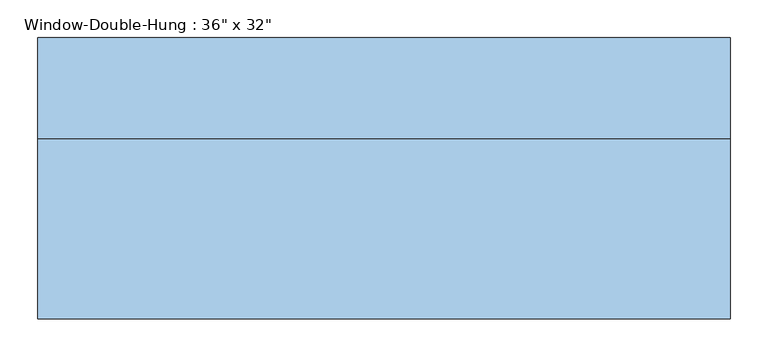
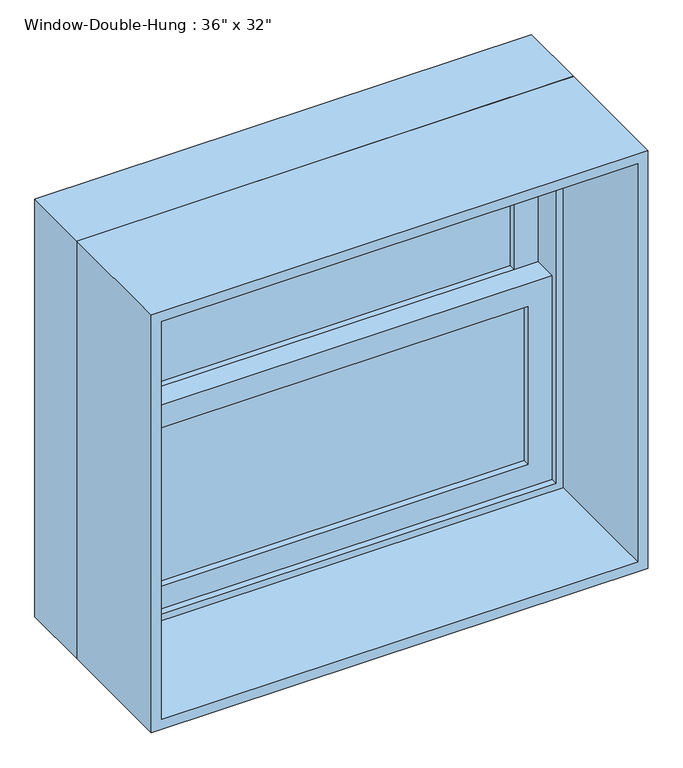
"""IFC4 building model written with IfcOpenShell, lengths in millimetres: window geometry."""

from ifc_helpers import new_model, si_unit, frame, origin, place, context, project, spatial, polyline, outline, extrude, source, transform, mapped, element, save


def window_e999161c(model_context):
    return source(origin(), model_context, "Body", "SweptSolid", [
        extrude(outline(polyline([(381.0, 106.3625), (381.0, 100.0125), (-381.0, 100.0125), (-381.0, 106.3625), (381.0, 106.3625)])), frame((0.0, 0.0, 990.6), z_axis=(0.0, 0.0, 1.0), x_axis=(1.0, 0.0, 0.0)), (0.0, 0.0, 1.0), 307.975),
        extrude(outline(polyline([(-381.0, 93.6625), (381.0, 93.6625), (381.0, 87.3125), (-381.0, 87.3125), (-381.0, 93.6625)])), frame((0.0, 0.0, 990.6), z_axis=(0.0, 0.0, 1.0), x_axis=(1.0, 0.0, 0.0)), (0.0, 0.0, 1.0), 307.975),
        extrude(outline(polyline([(381.0, 150.8125), (381.0, 144.4625), (-381.0, 144.4625), (-381.0, 150.8125), (381.0, 150.8125)])), frame((0.0, 0.0, 1343.025), z_axis=(0.0, 0.0, 1.0), x_axis=(1.0, 0.0, 0.0)), (0.0, 0.0, 1.0), 307.975),
        extrude(outline(polyline([(-381.0, 138.1125), (381.0, 138.1125), (381.0, 131.7625), (-381.0, 131.7625), (-381.0, 138.1125)])), frame((0.0, 0.0, 1343.025), z_axis=(0.0, 0.0, 1.0), x_axis=(1.0, 0.0, 0.0)), (0.0, 0.0, 1.0), 307.975),
        extrude(outline(polyline([(1343.025, -425.45), (946.15, -425.45), (946.15, 425.45), (1343.025, 425.45), (1343.025, -425.45)]), holes=[polyline([(1298.575, 381.0), (990.6, 381.0), (990.6, -381.0), (1298.575, -381.0), (1298.575, 381.0)])]), frame((0.0, 74.6125, 0.0), z_axis=(0.0, 1.0, 0.0), x_axis=(0.0, 0.0, 1.0)), (0.0, 0.0, 1.0), 44.45),
        extrude(outline(polyline([(1695.45, -425.45), (1298.575, -425.45), (1298.575, 425.45), (1695.45, 425.45), (1695.45, -425.45)]), holes=[polyline([(1651.0, 381.0), (1343.025, 381.0), (1343.025, -381.0), (1651.0, -381.0), (1651.0, 381.0)])]), frame((0.0, 119.0625, 0.0), z_axis=(0.0, 1.0, 0.0), x_axis=(0.0, 0.0, 1.0)), (0.0, 0.0, 1.0), 44.45),
        extrude(outline(polyline([(1727.2, -457.2), (914.4, -457.2), (914.4, 457.2), (1727.2, 457.2), (1727.2, -457.2)]), holes=[polyline([(1695.45, 425.45), (946.15, 425.45), (946.15, -425.45), (1695.45, -425.45), (1695.45, 425.45)])]), frame((0.0, 61.9125, 0.0), z_axis=(0.0, 1.0, 0.0), x_axis=(0.0, 0.0, 1.0)), (0.0, 0.0, 1.0), 133.35),
        extrude(outline(polyline([(1727.2, 457.2), (1727.2, -457.2), (914.4, -457.2), (914.4, 457.2), (1727.2, 457.2)]), holes=[polyline([(1708.15, 438.15), (933.45, 438.15), (933.45, -438.15), (1708.15, -438.15), (1708.15, 438.15)])]), frame((0.0, -176.2125, 0.0), z_axis=(0.0, 1.0, 0.0), x_axis=(0.0, 0.0, 1.0)), (0.0, 0.0, 1.0), 238.125),
    ])


if __name__ == "__main__":
    model = new_model("IFC4")
    model_context = context("Model", 3, world=origin())
    ifc_project = project(units=[si_unit("LENGTHUNIT", "METRE", prefix="MILLI")], contexts=[model_context])
    site = spatial("IfcSite", under=ifc_project)
    building = spatial("IfcBuilding", under=site)
    placement = place(None, origin())
    window_shape = window_e999161c(model_context)
    element("IfcWindow", 1, ObjectType="Window-Double-Hung : 36\" x 32\"", at=placement, inside=building, context=model_context, shape_type="MappedRepresentation", body=[
        mapped(window_shape, transform((0.0, 0.0, 0.0), x_axis=(1.0, 0.0, 0.0), y_axis=(0.0, 1.0, 0.0), z_axis=(0.0, 0.0, 1.0))),
    ])
    save(model, "model.ifc")

# Revit data of these elements
# Type "Window-Double-Hung : 36\" x 32\""
#   Type Mark = "19"
#   Fire Rating = "0.5h"
#   Construction Type Id = "DG-DR"
#   Assembly Code = "B2020100"
#   Analytic Construction = "Double glazing - domestic"
#   Wall Thickness [instance default] = 0' - 6"
#   Window Inset [instance default] = 0' - 0"
#   Visual Light Transmittance = 0.81
#   Thermal Resistance (R) = 1.8146 (h·ft²·°F)/BTU
#   Solar Heat Gain Coefficient = 0.76
#   Muntin Width = 2' - 6"
#   Muntin Height = 1' - 0 1/8"
#   Interior Wall Closure [instance default] = 0' - 1 1/2"
#   Rough Width = 3' - 0 1/2"
#   Rough Height = 2' - 8 1/2"
#   Frame Extension [instance default] = 0' - 1 1/4"
#   Exterior Wall Closure [instance default] = 0' - 0 1/2"
#   Extension Jamb [instance default] = 0' - 1 1/2"
#   Heat Transfer Coefficient (U) = 0.5511 BTU/(h·ft²·°F)
#   Height = 2' - 8"
#   Width = 3' - 0"
#   Top Muntin Visibility = yes
#   Indicator Visibility [instance default] = yes
#   Extension Jamb Visibility [instance default] = yes
#   Interior Trim Visibility [instance default] = yes
#   Exterior Trim Visibility [instance default] = yes
#   Define Thermal Properties by = 1
#   Bottom Muntin Visibility = yes
#   Muntin Pattern = Muntin Pattern_2x2 : Muntin Pattern_2x2
#   Interior Trim Material = Wood - Stained
#   Interior Trim = Trim-Window-Interior-Flat : Picture Frame
#   Exterior Trim Material = Clad - White
#   Exterior Trim = Trim-Window-Exterior-Flat : with Sill
#   Glass Panel Material = Glass
#   Exterior Frame Material = Clad - White
#   Interior Frame Material = Wood - Stained
#   Wall Closure = (empty or 0)
# Element 1 (IfcWindow, "Window-Double-Hung : 36\" x 32\"")
#   Wall Thickness = 1' - 1 7/8"
#   Extension Jamb = 0' - 9 3/8"
#   Materials on its faces: "Wood - Stained", "Glass", "Clad - White"
# Materials
#   "Wood - Stained": class "Wood", colour RGB 224 178 126, transparency 0, Cost = 0
#   "Clad - White": class "Wood", colour RGB 242 242 238, transparency 0, Cost = 0
#   "Glass": class "Glass", colour RGB 0 128 192, transparency 0.75, Description = "Soda Lime Glass", Cost = 0
